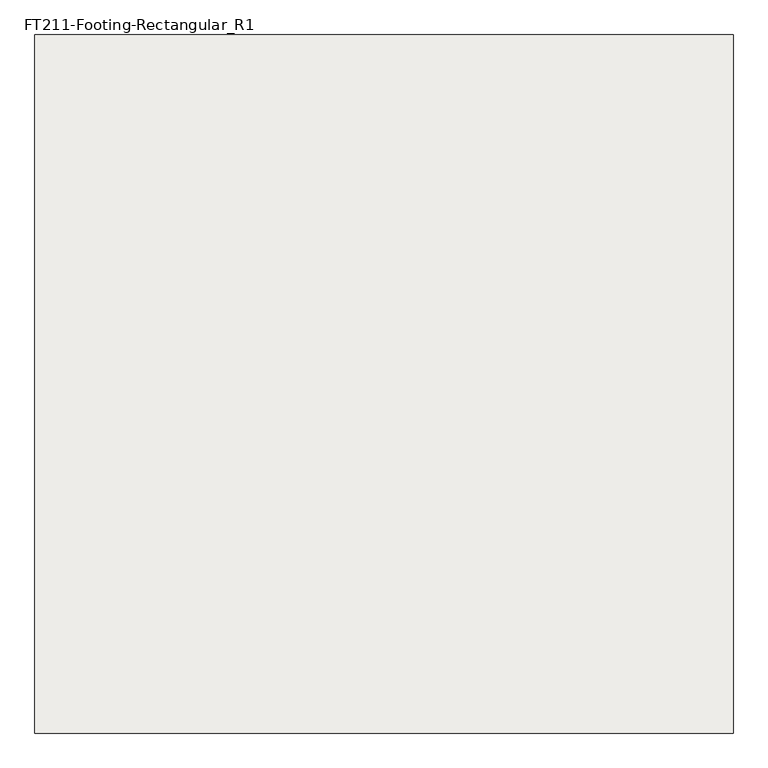
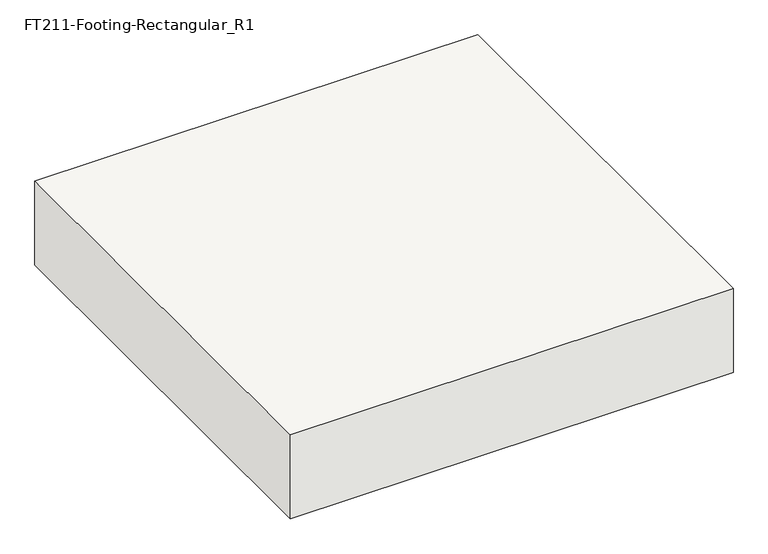
"""IFC4 building model written with IfcOpenShell, lengths in millimetres: slab geometry, FT211-Footing-Rectangular_R1 : H_SF_ACF_W2000xL2000xT400_Bitumen."""

from ifc_helpers import new_model, si_unit, frame, origin, place, context, project, spatial, polyline, outline, extrude, source, transform, mapped, element, save


def ft211_footing_rectangular_r1_4779d05c(model_context):
    return source(origin(), model_context, "Body", "SweptSolid", [
        extrude(outline(polyline([(1000.0, 1000.0), (1000.0, -1000.0), (-1000.0, -1000.0), (-1000.0, 1000.0), (1000.0, 1000.0)])), frame((0.0, 0.0, -400.0), z_axis=(0.0, 0.0, 1.0), x_axis=(1.0, 0.0, 0.0)), (0.0, 0.0, 1.0), 400.0),
    ])


if __name__ == "__main__":
    model = new_model("IFC4")
    model_context = context("Model", 3, world=origin())
    ifc_project = project(units=[si_unit("LENGTHUNIT", "METRE", prefix="MILLI")], contexts=[model_context])
    site = spatial("IfcSite", under=ifc_project)
    building = spatial("IfcBuilding", under=site)
    placement = place(None, origin())
    ft211_footing_rectangular_r1_shape = ft211_footing_rectangular_r1_4779d05c(model_context)
    element("IfcSlab", 1, ObjectType="FT211-Footing-Rectangular_R1 : H_SF_ACF_W2000xL2000xT400_Bitumen", at=placement, inside=building, context=model_context, shape_type="MappedRepresentation", body=[
        mapped(ft211_footing_rectangular_r1_shape, transform((0.0, 0.0, 0.0), x_axis=(1.0, 0.0, 0.0), y_axis=(0.0, 1.0, 0.0), z_axis=(0.0, 0.0, 1.0))),
    ])
    save(model, "model.ifc")

# Revit data of these elements
# Type "FT211-Footing-Rectangular_R1 : H_SF_ACF_W2000xL2000xT400_Bitumen"
#   Top bar = "D25@300"
#   Description = "UG Shallow Foundation"
#   Bottom bar = "D20@300"
#   Width = 2000.000 mm
#   Length = 2000.000 mm
#   Foundation Thickness = 400.000 mm
#   Structural Material [instance default] = none
#   Assembly Code = ""
